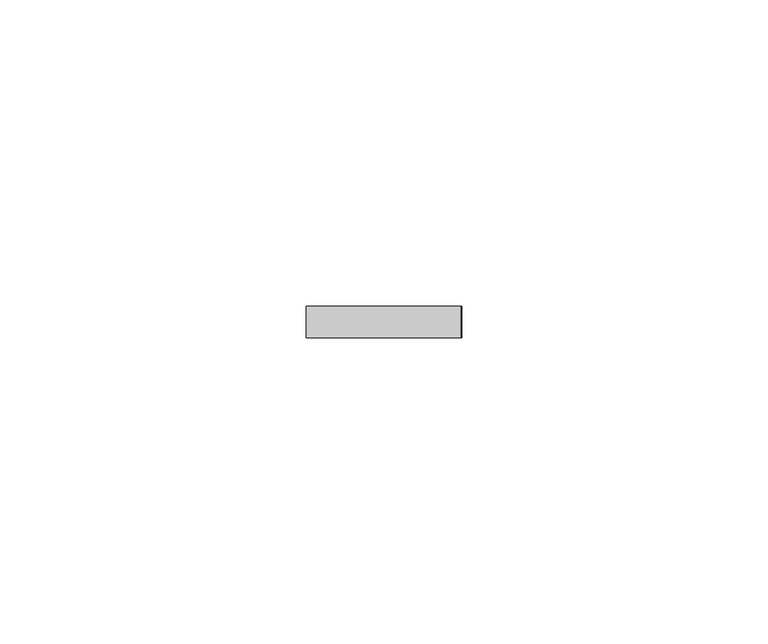
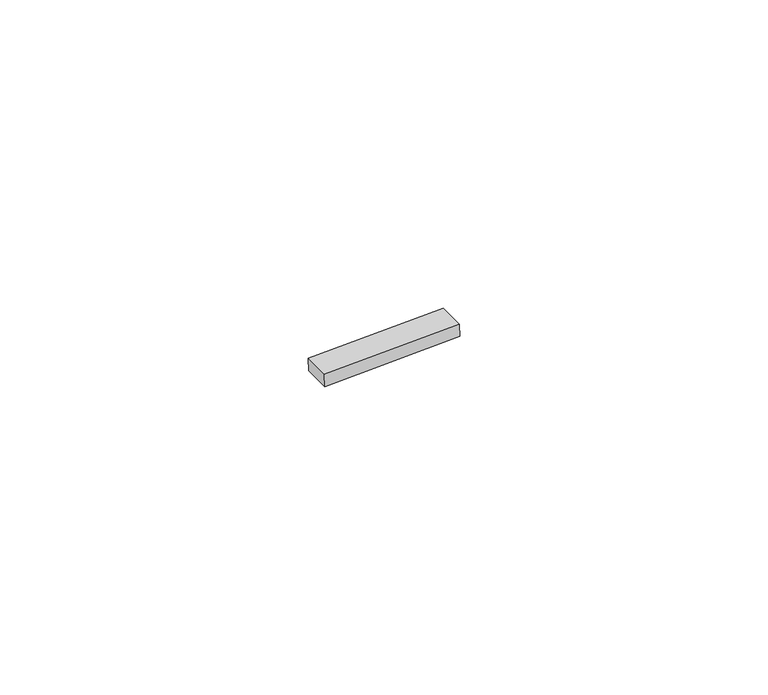
"""IFC4 building model written with IfcOpenShell, lengths in millimetres: proxy geometry, Inner panel:Inner panel:1:Inner panel:1 : Inner panel:Inner panel:300324:2:Inner panel:1:Inner panel:1 : Inner panel:Inner panel:300324:2 : Inner panel:Inner panel:1:Inner panel:1 : Inner panel:Inner panel:300324:300043:173 : Inner panel:Inner panel:1:Inner panel:1 : Inner panel:Inner panel:300324:2:Inner panel:1:Inner panel:1 : Inner panel:Inner panel:300324:2 : Inner panel:Inner panel:1:Inner panel:1 : Inner panel:Inner panel:300324:300043:308120."""

from ifc_helpers import new_model, si_unit, frame, origin, place, context, project, spatial, polyline, outline, extrude, source, transform, mapped, element, save


def generic_models_8fa1ce6f(model_context):
    return source(origin(), model_context, "Body", "SweptSolid", [
        extrude(outline(polyline([(0.0, -25.4), (0.0, 0.0), (5.213809, 0.0), (5.213809, -25.4), (0.0, -25.4)])), frame((560380.9331581, -565400.507991, 3950.5346612), z_axis=(-0.041630544712223896, 0.0, 0.9991330730923502), x_axis=(0.0, -1.0, 0.0)), (0.0, 0.0, 1.0), 2.4763745),
    ])


if __name__ == "__main__":
    model = new_model("IFC4")
    model_context = context("Model", 3, world=origin())
    ifc_project = project(units=[si_unit("LENGTHUNIT", "METRE", prefix="MILLI")], contexts=[model_context])
    site = spatial("IfcSite", under=ifc_project)
    building = spatial("IfcBuilding", under=site)
    placement = place(None, origin())
    generic_models_shape = generic_models_8fa1ce6f(model_context)
    element("IfcBuildingElementProxy", 1, Name="Inner panel:Inner panel:1:Inner panel:1 : Inner panel:Inner panel:300324:2:Inner panel:1:Inner panel:1 : Inner panel:Inner panel:300324:2 : Inner panel:Inner panel:1:Inner panel:1 : Inner panel:Inner panel:300324:300043:173 : Inner panel:Inner panel:1:Inner panel:1 : Inner panel:Inner panel:300324:2:Inner panel:1:Inner panel:1 : Inner panel:Inner panel:300324:2 : Inner panel:Inner panel:1:Inner panel:1 : Inner panel:Inner panel:300324:300043:308120", ObjectType="Inner panel:Inner panel:1:Inner panel:1 : Inner panel:Inner panel:300324:2:Inner panel:1:Inner panel:1 : Inner panel:Inner panel:300324:2 : Inner panel:Inner panel:1:Inner panel:1 : Inner panel:Inner panel:300324:300043:173 : Inner panel:Inner panel:1:Inner panel:1 : Inner panel:Inner panel:300324:2:Inner panel:1:Inner panel:1 : Inner panel:Inner panel:300324:2 : Inner panel:Inner panel:1:Inner panel:1 : Inner panel:Inner panel:300324:300043:308120", at=placement, inside=building, context=model_context, shape_type="MappedRepresentation", body=[
        mapped(generic_models_shape, transform((0.0, 0.0, 0.0), x_axis=(1.0, 0.0, 0.0), y_axis=(0.0, 1.0, 0.0), z_axis=(0.0, 0.0, 1.0))),
    ])
    save(model, "model.ifc")

# Revit data of these elements
# Type "Inner panel:Inner panel:1:Inner panel:1 : Inner panel:Inner panel:300324:2:Inner panel:1:Inner panel:1 : Inner panel:Inner panel:300324:2 : Inner panel:Inner panel:1:Inner panel:1 : Inner panel:Inner panel:300324:300043:173 : Inner panel:Inner panel:1:Inner panel:1 : Inner panel:Inner panel:300324:2:Inner panel:1:Inner panel:1 : Inner panel:Inner panel:300324:2 : Inner panel:Inner panel:1:Inner panel:1 : Inner panel:Inner panel:300324:300043:308120"
#   NameOverride = "Inner panel:Inner panel:1:Inner panel:1 : Inner panel:Inner panel:300324:2:Inner panel:1:Inner panel:1 : Inner panel:Inner panel:300324:2 : Inner panel:Inner panel:1:Inner panel:1 : Inner panel:Inner panel:300324:300043:308120"
#   ObjectTypeOverride = "Inner panel:1:Inner panel:1 : Inner panel:Inner panel:300324:2 : Inner panel:Inner panel:1:Inner panel:1 : Inner panel:Inner panel:300324:300043"
#   Reference = "Inner panel"
#   Tag = "308120"
# Element 1 (IfcBuildingElementProxy, "Inner panel:Inner panel:1:Inner panel:1 : Inner panel:Inner panel:300324:2:Inner panel:1:Inner panel:1 : Inner panel:Inner panel:300324:2 : Inner panel:Inner panel:1:Inner panel:1 : Inner panel:Inner panel:300324:300043:173 : Inner panel:Inner panel:1:Inner panel:1 : Inner panel:Inner panel:300324:2:Inner panel:1:Inner panel:1 : Inner panel:Inner panel:300324:2 : Inner panel:Inner panel:1:Inner panel:1 : Inner panel:Inner panel:300324:300043:308120")
#   Materials on its faces: "AT CLIP - 1\" WIDE NON ABSORBENT, WEATHER-RESISTANT NEOPRENE/EPDM/SBR FOAM"
# Materials
#   "AT CLIP - 1\" WIDE NON ABSORBENT, WEATHER-RESISTANT NEOPRENE/EPDM/SBR FOAM": class "Generic", colour RGB 85 85 85, transparency 0, Cost = 0
